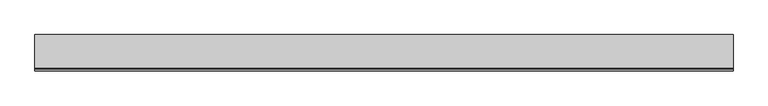
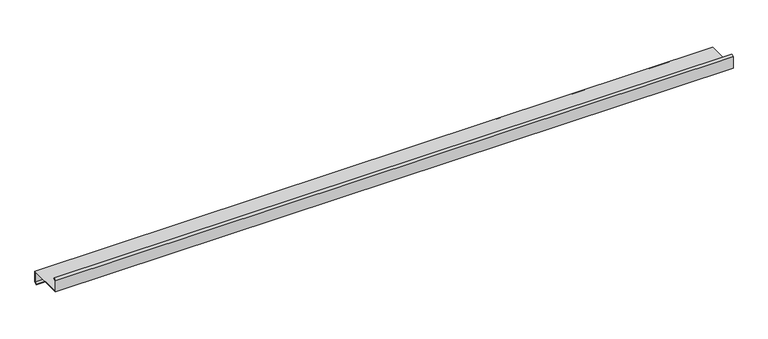
"""IFC4 building model written with IfcOpenShell, lengths in millimetres: proxy geometry, Generic Models 7:Generic Models 1:337419:Generic Models 1:337419 : Generic Models 7:Generic Models 1:337419:22 : Generic Models 7:Generic Models 1:337419:Generic Models 1:337419 : Generic Models 7:Generic Models 1:337419:301336."""

from ifc_helpers import new_model, si_unit, frame, origin, place, context, project, spatial, polyline, outline, extrude, source, transform, mapped, element, save


def generic_models_603024da(model_context):
    return source(origin(), model_context, "Body", "SweptSolid", [
        extrude(outline(polyline([(-536811.2913358, 8577.2625), (-536811.2913358, 8662.9863373), (-536796.8843797, 8675.0752089), (-536794.9124449, 8673.103274), (-536808.5132108, 8661.6908763), (-536808.5132108, 8580.040625), (-536557.2913358, 8580.040625), (-536557.2913358, 8500.6644623), (-536571.8844825, 8488.4193583), (-536573.8564173, 8490.3912932), (-536560.0694608, 8501.9599233), (-536560.0694608, 8577.2625), (-536811.2913358, 8577.2625)])), frame((591306.0367242, 0.0, 0.0), z_axis=(1.0, 0.0, 0.0), x_axis=(0.0, 1.0, 0.0)), (0.0, 0.0, 1.0), 4876.8),
    ])


if __name__ == "__main__":
    model = new_model("IFC4")
    model_context = context("Model", 3, world=origin())
    ifc_project = project(units=[si_unit("LENGTHUNIT", "METRE", prefix="MILLI")], contexts=[model_context])
    site = spatial("IfcSite", under=ifc_project)
    building = spatial("IfcBuilding", under=site)
    placement = place(None, origin())
    generic_models_shape = generic_models_603024da(model_context)
    element("IfcBuildingElementProxy", 1, Name="Generic Models 7:Generic Models 1:337419:Generic Models 1:337419 : Generic Models 7:Generic Models 1:337419:22 : Generic Models 7:Generic Models 1:337419:Generic Models 1:337419 : Generic Models 7:Generic Models 1:337419:301336", ObjectType="Generic Models 7:Generic Models 1:337419:Generic Models 1:337419 : Generic Models 7:Generic Models 1:337419:22 : Generic Models 7:Generic Models 1:337419:Generic Models 1:337419 : Generic Models 7:Generic Models 1:337419:301336", at=placement, inside=building, context=model_context, shape_type="MappedRepresentation", body=[
        mapped(generic_models_shape, transform((0.0, 0.0, 0.0), x_axis=(1.0, 0.0, 0.0), y_axis=(0.0, 1.0, 0.0), z_axis=(0.0, 0.0, 1.0))),
    ])
    save(model, "model.ifc")

# Revit data of these elements
# Type "Generic Models 7:Generic Models 1:337419:Generic Models 1:337419 : Generic Models 7:Generic Models 1:337419:22 : Generic Models 7:Generic Models 1:337419:Generic Models 1:337419 : Generic Models 7:Generic Models 1:337419:301336"
#   NameOverride = "Generic Models 7:Generic Models 1:337419:Generic Models 1:337419 : Generic Models 7:Generic Models 1:337419:301336"
#   ObjectTypeOverride = "Generic Models 1:337419 : Generic Models 7:Generic Models 1:337419"
#   Reference = "Generic Models 1"
#   Tag = "301336"
# Element 1 (IfcBuildingElementProxy, "Generic Models 7:Generic Models 1:337419:Generic Models 1:337419 : Generic Models 7:Generic Models 1:337419:22 : Generic Models 7:Generic Models 1:337419:Generic Models 1:337419 : Generic Models 7:Generic Models 1:337419:301336")
#   Materials on its faces: "'ZEE' SECTION (8.0x3.5Z - SEE STRUCT. DWGS)"
# Materials
#   "'ZEE' SECTION (8.0x3.5Z - SEE STRUCT. DWGS)": class "Unassigned", colour RGB 210 209 208, transparency 0, Keynote = "M05121300.02", Cost = 0
